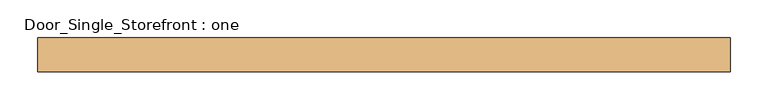
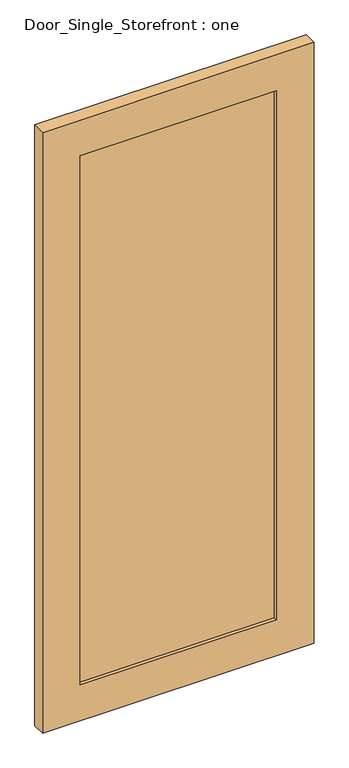
"""IFC4 building model written with IfcOpenShell, lengths in millimetres: door geometry, Door_Single_Storefront : one."""

from ifc_helpers import new_model, si_unit, frame, origin, place, context, project, spatial, polyline, outline, extrude, source, transform, mapped, element, save


def door_single_storefront_one_7b594b39(model_context):
    return source(origin(), model_context, "Body", "SweptSolid", [
        extrude(outline(polyline([(330.2, -6.35), (-330.2, -6.35), (-330.2, 12.7), (330.2, 12.7), (330.2, -6.35)])), frame((0.0, 0.0, 127.0), z_axis=(0.0, 0.0, 1.0), x_axis=(1.0, 0.0, 0.0)), (0.0, 0.0, 1.0), 1881.1875),
        extrude(outline(polyline([(2135.1875, -457.2), (0.0, -457.2), (0.0, 457.2), (2135.1875, 457.2), (2135.1875, -457.2)]), holes=[polyline([(127.0, 330.2), (127.0, -330.2), (2008.1875, -330.2), (2008.1875, 330.2), (127.0, 330.2)])]), frame((0.0, -19.05, 0.0), z_axis=(0.0, 1.0, 0.0), x_axis=(0.0, 0.0, 1.0)), (0.0, 0.0, 1.0), 44.45),
    ])


if __name__ == "__main__":
    model = new_model("IFC4")
    model_context = context("Model", 3, world=origin())
    ifc_project = project(units=[si_unit("LENGTHUNIT", "METRE", prefix="MILLI")], contexts=[model_context])
    site = spatial("IfcSite", under=ifc_project)
    building = spatial("IfcBuilding", under=site)
    placement = place(None, origin())
    door_single_storefront_one_shape = door_single_storefront_one_7b594b39(model_context)
    element("IfcDoor", 1, ObjectType="Door_Single_Storefront : one", at=placement, inside=building, context=model_context, shape_type="MappedRepresentation", body=[
        mapped(door_single_storefront_one_shape, transform((0.0, 0.0, 0.0), x_axis=(1.0, 0.0, 0.0), y_axis=(0.0, 1.0, 0.0), z_axis=(0.0, 0.0, 1.0))),
    ])
    save(model, "model.ifc")

# Revit data of these elements
# Type "Door_Single_Storefront : one"
#   Type Mark = "29"
#   Analytic Construction = "<None>"
#   Stile_Width = 0' - 5"
#   Door_Thickness = 0' - 1 3/4"
#   Door_Offset = 0' - 1"
#   Glass_Material = ALUM. STOREFRONT W/ INSULATED GLAZING
#   Frame_Material = Aluminum
#   Function = (empty or 0)
# Element 1 (IfcDoor, "Door_Single_Storefront : one")
#   Materials on its faces: "Aluminum", "ALUM. STOREFRONT W/ INSULATED GLAZING"
# Materials
#   "ALUM. STOREFRONT W/ INSULATED GLAZING": class "Glass", colour RGB 196 205 210, transparency 0.85, Description = "Soda Lime Glass", Cost = 0
#   "Aluminum": class "Metal", colour RGB 244 244 244, transparency 0, Description = "Aluminum 6061", Cost = 0
